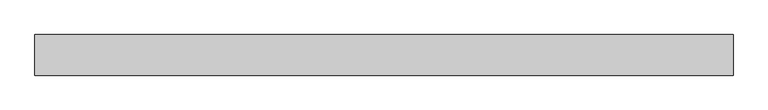
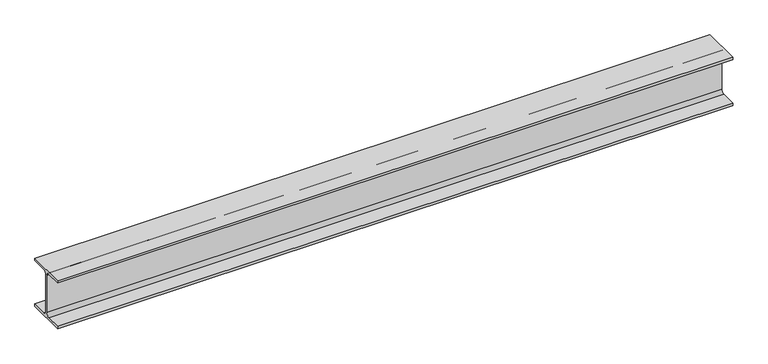
"""IFC4 building model written with IfcOpenShell, lengths in millimetres: beam geometry, 0912_Steel Framing_H-KSD3502 : H_SB_ASB_H-194x150x6x9."""

from ifc_helpers import new_model, si_unit, point, frame, frame_2d, origin, place, context, project, spatial, polyline, circle_curve, trimmed, segment, composite_curve, outline, extrude, source, transform, mapped, element, save


def beam_70c5134d(model_context):
    return source(origin(), model_context, "Body", "SweptSolid", [
        extrude(outline(composite_curve([segment(polyline([(75.0, -88.0), (75.0, -97.0), (-75.0, -97.0), (-75.0, -88.0), (-16.0, -88.0)]), True, "CONTINUOUS"), segment(trimmed(circle_curve(frame_2d((-16.0, -75.0)), 13.0), [point((-16.0, -88.0))], [point((-3.0, -75.0))], True, "CARTESIAN"), True, "CONTINUOUS"), segment(polyline([(-3.0, -75.0), (-3.0, 75.0)]), True, "CONTINUOUS"), segment(trimmed(circle_curve(frame_2d((-16.0, 75.0)), 13.0), [point((-3.0, 75.0))], [point((-16.0, 88.0))], True, "CARTESIAN"), True, "CONTINUOUS"), segment(polyline([(-16.0, 88.0), (-75.0, 88.0), (-75.0, 97.0), (75.0, 97.0), (75.0, 88.0), (16.0, 88.0)]), True, "CONTINUOUS"), segment(trimmed(circle_curve(frame_2d((16.0, 75.0)), 13.0), [point((16.0, 88.0))], [point((3.0, 75.0))], True, "CARTESIAN"), True, "CONTINUOUS"), segment(polyline([(3.0, 75.0), (3.0, -75.0)]), True, "CONTINUOUS"), segment(trimmed(circle_curve(frame_2d((16.0, -75.0)), 13.0), [point((3.0, -75.0))], [point((16.0, -88.0))], True, "CARTESIAN"), True, "CONTINUOUS"), segment(polyline([(16.0, -88.0), (75.0, -88.0)]), True, "CONTINUOUS")], self_intersect=False)), frame((-1265.0, 0.0, 0.0), z_axis=(1.0, 0.0, 0.0), x_axis=(0.0, 1.0, 0.0)), (0.0, 0.0, 1.0), 2578.0465428),
    ])


if __name__ == "__main__":
    model = new_model("IFC4")
    model_context = context("Model", 3, world=origin())
    ifc_project = project(units=[si_unit("LENGTHUNIT", "METRE", prefix="MILLI")], contexts=[model_context])
    site = spatial("IfcSite", under=ifc_project)
    building = spatial("IfcBuilding", under=site)
    placement = place(None, origin())
    beam_shape = beam_70c5134d(model_context)
    element("IfcBeam", 1, ObjectType="0912_Steel Framing_H-KSD3502 : H_SB_ASB_H-194x150x6x9", at=placement, inside=building, context=model_context, shape_type="MappedRepresentation", body=[
        mapped(beam_shape, transform((0.0, 0.0, 0.0), x_axis=(1.0, 0.0, 0.0), y_axis=(0.0, 1.0, 0.0), z_axis=(0.0, 0.0, 1.0))),
    ])
    save(model, "model.ifc")

# Revit data of these elements
# Type "0912_Steel Framing_H-KSD3502 : H_SB_ASB_H-194x150x6x9"
#   H_WM Code_1 = "S01AA002-00001 | Main Steel Structure Fabrication Work | Shelter/Building | Medium Steel - Standard (90KG/M>Weight≥30KG/M) | Material: (   )"
#   H_WM Code_2 = "S03AA028-00001 | Main Steel Structure Erection Work | Shelter/Building | Medium Steel (90KG/M>Weight≥30KG/M) | Material: (   )"
#   H_WM Code_3 = "S01AA010-00001 | Main Steel Structure Fabrication Work | Shelter/Building | Steel Painting/Coating | for Non-Fireproofed Steel Surface, Surface Preparation, Primer, Second & Final Coat | Material: (   )"
#   H_Q'ty Cal Type Tag = "SB-Q2"
#   Width = 15.0 cm
#   Web Thickness = 0.6 cm
#   Web Fillet = 1.3 cm
#   Warping Constant = 43316.0 cm⁶
#   W = 0
#   Torsional Moment of Inertia = 8.622 cm⁴
#   Section Area = 39.01 cm²
#   Plastic Modulus weak axis = 104.0 cm³
#   Plastic Modulus strong axis = 309.0 cm³
#   Perimeter = 0.95 m²/m
#   Nominal Weight = 30.60 kgf/m
#   Moment of Inertia weak axis = 507.00 cm⁴
#   Moment of Inertia strong axis = 2690.00 cm⁴
#   Height = 19.4 cm
#   Flange Thickness = 0.9 cm
#   Elastic Modulus weak axis = 67.6 cm³
#   Elastic Modulus strong axis = 277.0 cm³
#   Centroid Vertical = 9.7 cm
#   Centroid Horizontal = 7.5 cm
#   Ix = 26900000
#   Length [instance default] = 1.5240 m
#   Zx = 309000
#   b = 0.1500 m
#   h = 0.1940 m
#   r = 0.0130 m
#   s = 0.0060 m
#   t = 0.0090 m
#   A = 0.003901 m²
#   Structural Material [instance default] = Steel, 45-345
#   Assembly Code = ""
# Element 1 (IfcBeam, "0912_Steel Framing_H-KSD3502 : H_SB_ASB_H-194x150x6x9")
#   Structural Material = none
# Materials
#   "Steel, 45-345": class "Metal", colour RGB 189 187 185, transparency 0, Description = "Steel 345 MPa", Cost = 0
